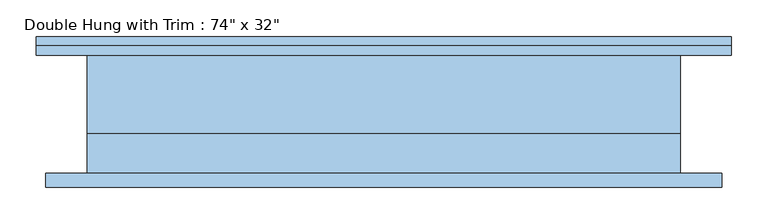
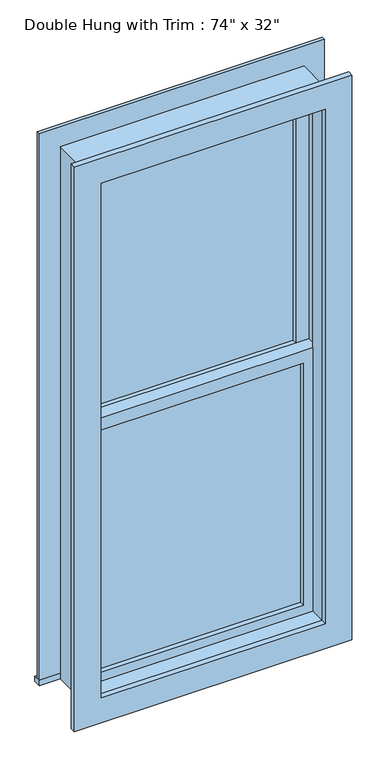
"""IFC4 building model written with IfcOpenShell, lengths in millimetres: window geometry."""

import ifcopenshell
import ifcopenshell.guid

model = None  # the IFC model being written
_history = None  # IfcOwnerHistory: only IFC2X3 demands one
_inside = {}  # id of a spatial element -> (the spatial element, [elements in it])
_under = {}  # id of a project, library or spatial element -> (it, [spatial elements below it])
_declared = {}  # id of a project -> (the project, [libraries it declares])
_typed = {}  # id of a type object -> (the type object, [elements of that type])
_made_of = {}  # id of a material, layer set ... -> (it, [elements and type objects made of it])


def new_model(schema):
    """Start an empty IFC model of exactly this schema.

    Asked for "IFC4X3", IfcOpenShell would pick the latest addendum, in which some entities
    have other attributes; the version numbers below select the first issue.
    IFC2X3 requires an IfcOwnerHistory on every rooted entity: one is made here for all.
    """
    global model, _history
    if schema == "IFC4X3":
        model = ifcopenshell.file(schema_version=(4, 3, 0, 0))
    else:
        model = ifcopenshell.file(schema=schema)
    _inside.clear()
    _under.clear()
    _declared.clear()
    _typed.clear()
    _made_of.clear()
    _history = None
    if model.schema == "IFC2X3":
        org = make("IfcOrganization", Name="unknown")
        user = make(
            "IfcPersonAndOrganization",
            ThePerson=make("IfcPerson", FamilyName="unknown"),
            TheOrganization=org,
        )
        app = make(
            "IfcApplication",
            ApplicationDeveloper=org,
            Version="unknown",
            ApplicationFullName="unknown",
            ApplicationIdentifier="unknown",
        )
        _history = make(
            "IfcOwnerHistory",
            OwningUser=user,
            OwningApplication=app,
            ChangeAction="ADDED",
            CreationDate=0,
        )
    return model


def make(cls, **values):
    """One entity of the class cls with the attributes given. An attribute that is None is left unset."""
    return model.create_entity(
        cls, **{name: value for name, value in values.items() if value is not None}
    )


def rooted(cls, **values):
    """An entity with a GlobalId (a new one), such as an element, a storey or a relation."""
    return make(cls, GlobalId=ifcopenshell.guid.new(), OwnerHistory=_history, **values)


def si_unit(unit_type, name, prefix=None):
    """IfcSIUnit, for example si_unit("LENGTHUNIT", "METRE", prefix="MILLI")."""
    return make("IfcSIUnit", UnitType=unit_type, Prefix=prefix, Name=name)


def assignment(units):
    """IfcUnitAssignment: the units of a project."""
    return None if units is None else make("IfcUnitAssignment", Units=units)


def point(xyz):
    """IfcCartesianPoint."""
    return None if xyz is None else make("IfcCartesianPoint", Coordinates=xyz)


def direction(xyz):
    """IfcDirection."""
    return None if xyz is None else make("IfcDirection", DirectionRatios=xyz)


def frame(location, z_axis=None, x_axis=None):
    """IfcAxis2Placement3D, a coordinate frame: its origin and axes. An axis left out is left unset."""
    return make(
        "IfcAxis2Placement3D",
        Location=point(location),
        Axis=direction(z_axis),
        RefDirection=direction(x_axis),
    )


def origin():
    """The frame at (0, 0, 0) with its axes left unset."""
    return frame((0.0, 0.0, 0.0))


def place(relative_to, where):
    """IfcLocalPlacement: puts the frame where relative to a parent placement (None: the world)."""
    return make(
        "IfcLocalPlacement", PlacementRelTo=relative_to, RelativePlacement=where
    )


def context(
    kind, dimensions, precision=None, world=None, true_north=None, identifier=None
):
    """IfcGeometricRepresentationContext, for example the 3D "Model" context."""
    return make(
        "IfcGeometricRepresentationContext",
        ContextIdentifier=identifier,
        ContextType=kind,
        CoordinateSpaceDimension=dimensions,
        Precision=precision,
        WorldCoordinateSystem=world,
        TrueNorth=true_north,
    )


def project(units=None, contexts=None):
    """IfcProject with its units and contexts."""
    return rooted(
        "IfcProject",
        Name="project",
        RepresentationContexts=contexts,
        UnitsInContext=assignment(units),
    )


def spatial(cls, under=None, at=None, **own):
    """A site, building, storey or space (cls), placed at a placement, below another one or the project."""
    s = rooted(cls, ObjectPlacement=at, **own)
    if under is not None:
        _under.setdefault(under.id(), (under, []))[1].append(s)
    return s


def polyline(points):
    """IfcPolyline through the points."""
    return make("IfcPolyline", Points=[point(p) for p in points])


def outline(outer, holes=None, kind="AREA"):
    """IfcArbitraryClosedProfileDef: a profile drawn as a closed curve; with holes, ...WithVoids."""
    if holes is None:
        return make("IfcArbitraryClosedProfileDef", ProfileType=kind, OuterCurve=outer)
    return make(
        "IfcArbitraryProfileDefWithVoids",
        ProfileType=kind,
        OuterCurve=outer,
        InnerCurves=holes,
    )


def extrude(swept, where, along, depth):
    """IfcExtrudedAreaSolid: the profile swept, set in the frame where, extruded along a direction by depth."""
    return make(
        "IfcExtrudedAreaSolid",
        SweptArea=swept,
        Position=where,
        ExtrudedDirection=direction(along),
        Depth=depth,
    )


def shape(context_of_items, identifier, shape_type, items):
    """IfcShapeRepresentation: the items that make up one representation, for example the "Body"."""
    return make(
        "IfcShapeRepresentation",
        ContextOfItems=context_of_items,
        RepresentationIdentifier=identifier,
        RepresentationType=shape_type,
        Items=items,
    )


def source(mapping_origin, context_of_items, identifier, shape_type, items):
    """IfcRepresentationMap: a shape defined once, which mapped items show again and again."""
    return make(
        "IfcRepresentationMap",
        MappingOrigin=mapping_origin,
        MappedRepresentation=shape(context_of_items, identifier, shape_type, items),
    )


def transform(
    local_origin,
    x_axis=None,
    y_axis=None,
    z_axis=None,
    scale=None,
    scale2=None,
    scale3=None,
    uniform=True,
):
    """IfcCartesianTransformationOperator3D, or its non-uniform kind. x_axis, y_axis, z_axis: its Axis1, 2, 3."""
    if uniform:
        return make(
            "IfcCartesianTransformationOperator3D",
            Axis1=direction(x_axis),
            Axis2=direction(y_axis),
            LocalOrigin=point(local_origin),
            Scale=scale,
            Axis3=direction(z_axis),
        )
    return make(
        "IfcCartesianTransformationOperator3DnonUniform",
        Axis1=direction(x_axis),
        Axis2=direction(y_axis),
        LocalOrigin=point(local_origin),
        Scale=scale,
        Axis3=direction(z_axis),
        Scale2=scale2,
        Scale3=scale3,
    )


def mapped(mapping_source, mapping_target):
    """IfcMappedItem: shows the shape of a source again, moved by a transform."""
    return make(
        "IfcMappedItem", MappingSource=mapping_source, MappingTarget=mapping_target
    )


def made_of(thing, what):
    """Note that an element or type object is made of a material, layer set ...; save() writes the relation."""
    if what is not None:
        _made_of.setdefault(what.id(), (what, []))[1].append(thing)
    return thing


def element(
    cls,
    number,
    at=None,
    inside=None,
    cuts=None,
    type_object=None,
    material=None,
    context=None,
    identifier="Body",
    shape_type=None,
    held_by="IfcProductDefinitionShape",
    body=None,
    shapes=None,
    **own,
):
    """One element of the class cls, such as IfcWall. Its Tag is "e" and its number.

    at: its placement. inside: the storey or other place that contains it. cuts: it is an
    opening in that element (IfcRelVoidsElement). A single representation is given by context,
    identifier, shape_type and body (its items); several are given by shapes. held_by: the class
    of the entity that holds the representations. save() writes the other relations.
    """
    e = rooted(cls, Tag="e%d" % number, ObjectPlacement=at, **own)
    if body is not None:
        shapes = [shape(context, identifier, shape_type, body)]
    if shapes is not None:
        e.Representation = make(held_by, Representations=shapes)
    if inside is not None:
        _inside.setdefault(inside.id(), (inside, []))[1].append(e)
    if cuts is not None:
        rooted(
            "IfcRelVoidsElement", RelatingBuildingElement=cuts, RelatedOpeningElement=e
        )
    if type_object is not None:
        _typed.setdefault(type_object.id(), (type_object, []))[1].append(e)
    return made_of(e, material)


def aggregate(whole, parts):
    """IfcRelAggregates: a whole, such as a stair, and the parts it consists of."""
    return rooted("IfcRelAggregates", RelatingObject=whole, RelatedObjects=parts)


def save(model, path):
    """Write the relations noted so far, then the file.

    IfcRelAggregates (storeys below a building ...), IfcRelContainedInSpatialStructure (elements
    in a storey), IfcRelDefinesByType, IfcRelAssociatesMaterial and IfcRelDeclares: one each for
    every whole, place, type object, material and project.
    """
    for whole, parts in _under.values():
        aggregate(whole, parts)
    for where, things in _inside.values():
        rooted(
            "IfcRelContainedInSpatialStructure",
            RelatedElements=things,
            RelatingStructure=where,
        )
    for kind, things in _typed.values():
        rooted("IfcRelDefinesByType", RelatedObjects=things, RelatingType=kind)
    for what, things in _made_of.values():
        rooted("IfcRelAssociatesMaterial", RelatedObjects=things, RelatingMaterial=what)
    for by, libraries in _declared.values():
        rooted("IfcRelDeclares", RelatingContext=by, RelatedDefinitions=libraries)
    model.write(path)


def window_c0b857e0(model_context):
    return source(origin(), model_context, "Body", "SweptSolid", [
        extrude(outline(polyline([(-342.9, 1.5875), (342.9, 1.5875), (342.9, -11.1125), (-342.9, -11.1125), (-342.9, 1.5875)])), frame((0.0, 0.0, 571.5), z_axis=(0.0, 0.0, 1.0), x_axis=(1.0, 0.0, 0.0)), (0.0, 0.0, 1.0), 854.075),
        extrude(outline(polyline([(1470.025, -387.35), (527.05, -387.35), (527.05, 387.35), (1470.025, 387.35), (1470.025, -387.35)]), holes=[polyline([(1425.575, -342.9), (1425.575, 342.9), (571.5, 342.9), (571.5, -342.9), (1425.575, -342.9)])]), frame((0.0, -26.9875, 0.0), z_axis=(0.0, 1.0, 0.0), x_axis=(0.0, 0.0, 1.0)), (0.0, 0.0, 1.0), 44.45),
        extrude(outline(polyline([(-476.25, 106.3625), (476.25, 106.3625), (476.25, 80.9625), (-476.25, 80.9625), (-476.25, 106.3625)])), frame((0.0, 0.0, 508.0), z_axis=(0.0, 0.0, 1.0), x_axis=(1.0, 0.0, 0.0)), (0.0, 0.0, 1.0), 19.05),
        extrude(outline(polyline([(2368.55, -387.35), (2368.55, 387.35), (527.05, 387.35), (527.05, 476.25), (2457.45, 476.25), (2457.45, -476.25), (527.05, -476.25), (527.05, -387.35), (2368.55, -387.35)])), frame((0.0, 80.9625, 0.0), z_axis=(0.0, 1.0, 0.0), x_axis=(0.0, 0.0, 1.0)), (0.0, 0.0, 1.0), 12.7),
        extrude(outline(polyline([(2444.75, 463.55), (2444.75, -463.55), (450.85, -463.55), (450.85, 463.55), (2444.75, 463.55)]), holes=[polyline([(2355.85, 374.65), (539.75, 374.65), (539.75, -374.65), (2355.85, -374.65), (2355.85, 374.65)])]), frame((0.0, -100.0125, 0.0), z_axis=(0.0, 1.0, 0.0), x_axis=(0.0, 0.0, 1.0)), (0.0, 0.0, 1.0), 19.05),
        extrude(outline(polyline([(342.9, 33.3375), (-342.9, 33.3375), (-342.9, 46.0375), (342.9, 46.0375), (342.9, 33.3375)])), frame((0.0, 0.0, 1470.025), z_axis=(0.0, 0.0, 1.0), x_axis=(1.0, 0.0, 0.0)), (0.0, 0.0, 1.0), 854.075),
        extrude(outline(polyline([(2368.55, -387.35), (1425.575, -387.35), (1425.575, 387.35), (2368.55, 387.35), (2368.55, -387.35)]), holes=[polyline([(2324.1, -342.9), (2324.1, 342.9), (1470.025, 342.9), (1470.025, -342.9), (2324.1, -342.9)])]), frame((0.0, 17.4625, 0.0), z_axis=(0.0, 1.0, 0.0), x_axis=(0.0, 0.0, 1.0)), (0.0, 0.0, 1.0), 44.45),
        extrude(outline(polyline([(2387.6, -406.4), (508.0, -406.4), (508.0, 406.4), (2387.6, 406.4), (2387.6, -406.4)]), holes=[polyline([(2355.85, -374.65), (2355.85, 374.65), (539.75, 374.65), (539.75, -374.65), (2355.85, -374.65)])]), frame((0.0, -80.9625, 0.0), z_axis=(0.0, 1.0, 0.0), x_axis=(0.0, 0.0, 1.0)), (0.0, 0.0, 1.0), 53.975),
        extrude(outline(polyline([(2387.6, 406.4), (2387.6, -406.4), (508.0, -406.4), (508.0, 406.4), (2387.6, 406.4)]), holes=[polyline([(2368.55, 387.35), (527.05, 387.35), (527.05, -387.35), (2368.55, -387.35), (2368.55, 387.35)])]), frame((0.0, -26.9875, 0.0), z_axis=(0.0, 1.0, 0.0), x_axis=(0.0, 0.0, 1.0)), (0.0, 0.0, 1.0), 107.95),
    ])


if __name__ == "__main__":
    model = new_model("IFC4")
    model_context = context("Model", 3, world=origin())
    ifc_project = project(units=[si_unit("LENGTHUNIT", "METRE", prefix="MILLI")], contexts=[model_context])
    site = spatial("IfcSite", under=ifc_project)
    building = spatial("IfcBuilding", under=site)
    placement = place(None, origin())
    window_shape = window_c0b857e0(model_context)
    element("IfcWindow", 1, ObjectType="Double Hung with Trim : 74\" x 32\"", at=placement, inside=building, context=model_context, shape_type="MappedRepresentation", body=[
        mapped(window_shape, transform((0.0, 0.0, 0.0), x_axis=(1.0, 0.0, 0.0), y_axis=(0.0, 1.0, 0.0), z_axis=(0.0, 0.0, 1.0))),
    ])
    save(model, "model.ifc")

# Revit data of these elements
# Type "Double Hung with Trim : 74\" x 32\""
#   Type Mark = "55"
#   COBie.Type.CreatedBy = "doug.wood@us.ibm.com"
#   COBie.Type.CreatedOn = "2016-04-14T02:07:26"
#   COBie.Type.Name = "Windows_Double Hung with Trim_74\" x 32\"_55"
#   COBie.Type.Category = "23-30 20 17 17 14 : Double-Hung Windows"
#   COBie.Type.Description = "Double Hung with Trim_74\" x 32\""
#   COBie.Type.Manufacturer = ""
#   COBie.Type.ModelNumber = ""
#   Construction Type Id = "GSP4R"
#   Assembly Code = "B2020100"
#   Analytic Construction = "1/8 in Pilkington single glazing"
#   COBie.Type.ReplacementCost = 0
#   Visual Light Transmittance = 0.9
#   Solar Heat Gain Coefficient = 0.78
#   Heat Transfer Coefficient (U) = 3.6886 W/(m²·K)
#   Height = 6' - 2"
#   Default Sill Height = 1' - 8"
#   Trim Projection - Ext. = 0' - 0 1/2"
#   Trim Projection - Int. = 0' - 0 3/4"
#   Trim Width - Exterior = 0' - 3 1/2"
#   Trim Width - Interior = 0' - 3 1/2"
#   Width = 2' - 8"
#   Window Inset = 0' - 0 3/4"
#   COBie.Type = no
#   Glass Pane Material = Glass
#   Sash Material = Sash - White
#   Trim Exterior Material = Trim - White
#   Trim Interior Material = Trim - White
#   Wall Closure = (empty or 0)
# Element 1 (IfcWindow, "Double Hung with Trim : 74\" x 32\"")
#   Materials on its faces: "Sash - White", "Trim - White", "Glass"
# Materials
#   "Glass": class "Glass", colour RGB 0 128 192, transparency 0.75, Description = "Soda Lime Glass", Cost = 0
#   "Sash - White": class "Wood", colour RGB 255 255 255, transparency 0, Cost = 0
#   "Trim - White": class "Wood", colour RGB 255 255 255, transparency 0, Cost = 0
